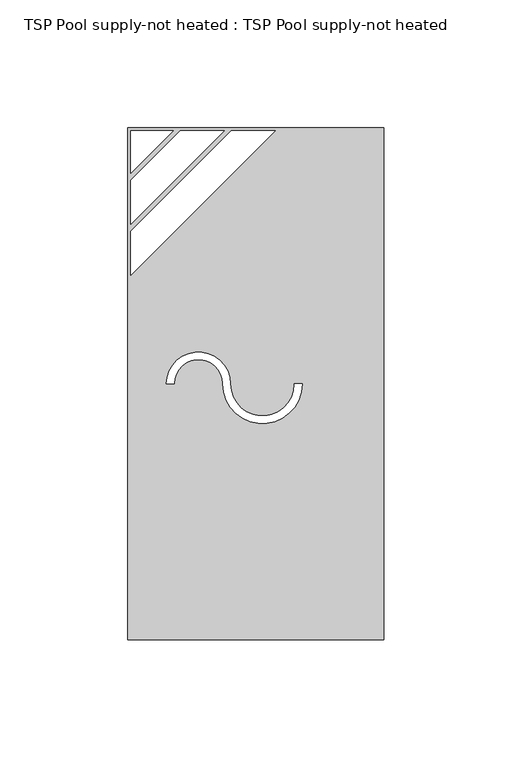
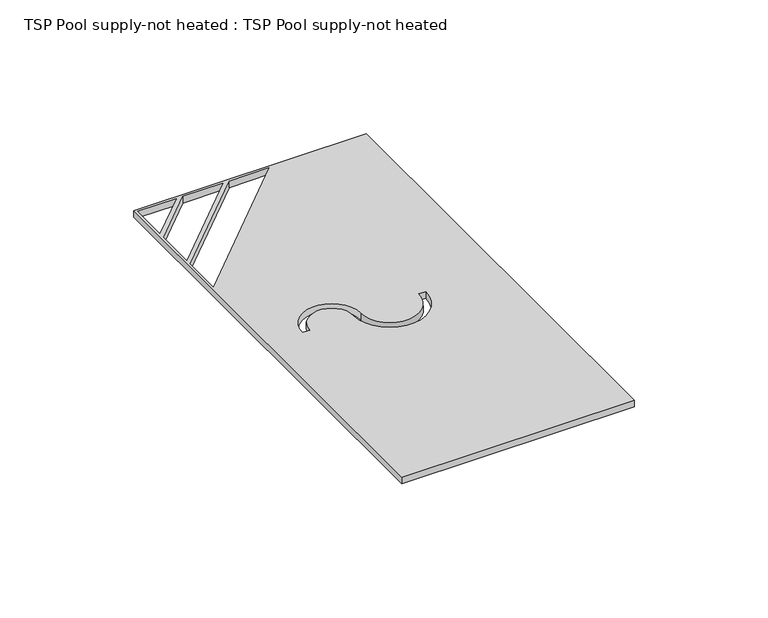
"""IFC4 building model written with IfcOpenShell, lengths in millimetres: proxy geometry, TSP Pool supply-not heated : TSP Pool supply-not heated."""

from ifc_helpers import new_model, si_unit, point, frame_2d, origin, origin_with_axes, place, context, project, spatial, polyline, circle_curve, trimmed, segment, composite_curve, outline, extrude, source, transform, mapped, element, save


def tsp_pool_supply_not_heated_tsp_pool_supply_not_heated_95d609e6(model_context):
    return source(origin(), model_context, "Body", "SweptSolid", [
        extrude(outline(polyline([(-100.0, 100.0), (0.0, 100.0), (0.0, -100.0), (-100.0, -100.0), (-100.0, 100.0)]), holes=[polyline([(-59.5857864, 99.0), (-99.0, 59.5857864), (-99.0, 42.4142136), (-42.4142136, 99.0), (-59.5857864, 99.0)]), polyline([(-99.0, 82.4142136), (-82.4142136, 99.0), (-99.0, 99.0), (-99.0, 82.4142136)]), polyline([(-99.0, 79.5857864), (-99.0, 62.4142136), (-62.4142136, 99.0), (-79.5857864, 99.0), (-99.0, 79.5857864)]), composite_curve([segment(trimmed(circle_curve(frame_2d((-72.5, 0.0)), 9.5), [point((-82.0, 0.0))], [point((-63.0, 0.0))], False, "CARTESIAN"), True, "CONTINUOUS"), segment(trimmed(circle_curve(frame_2d((-47.5, 0.0)), 15.5), [point((-63.0, 0.0))], [point((-32.0, 0.0))], True, "CARTESIAN"), True, "CONTINUOUS"), segment(polyline([(-32.0, 0.0), (-35.0, 0.0)]), True, "CONTINUOUS"), segment(trimmed(circle_curve(frame_2d((-47.5, 0.0)), 12.5), [point((-35.0, 0.0))], [point((-60.0, 0.0))], False, "CARTESIAN"), True, "CONTINUOUS"), segment(trimmed(circle_curve(frame_2d((-72.5, 0.0)), 12.5), [point((-60.0, 0.0))], [point((-85.0, 0.0))], True, "CARTESIAN"), True, "CONTINUOUS"), segment(polyline([(-85.0, 0.0), (-82.0, 0.0)]), True, "CONTINUOUS")], self_intersect=False)]), origin_with_axes(), (0.0, 0.0, 1.0), 3.0),
    ])


if __name__ == "__main__":
    model = new_model("IFC4")
    model_context = context("Model", 3, world=origin())
    ifc_project = project(units=[si_unit("LENGTHUNIT", "METRE", prefix="MILLI")], contexts=[model_context])
    site = spatial("IfcSite", under=ifc_project)
    building = spatial("IfcBuilding", under=site)
    placement = place(None, origin())
    tsp_pool_supply_not_heated_tsp_pool_supply_not_heated_shape = tsp_pool_supply_not_heated_tsp_pool_supply_not_heated_95d609e6(model_context)
    element("IfcBuildingElementProxy", 1, Name="TSP Pool supply-not heated : TSP Pool supply-not heated", ObjectType="TSP Pool supply-not heated : TSP Pool supply-not heated", at=placement, inside=building, context=model_context, shape_type="MappedRepresentation", body=[
        mapped(tsp_pool_supply_not_heated_tsp_pool_supply_not_heated_shape, transform((0.0, 0.0, 0.0), x_axis=(1.0, 0.0, 0.0), y_axis=(0.0, 1.0, 0.0), z_axis=(0.0, 0.0, 1.0))),
    ])
    save(model, "model.ifc")

# Revit data of these elements
# Type "TSP Pool supply-not heated : TSP Pool supply-not heated"
#   Model = "TSP_ELECSPSTD"
#   Default Elevation = 0
# Element 1 (IfcBuildingElementProxy, "TSP Pool supply-not heated : TSP Pool supply-not heated")
#   Materials on its faces: "Plastic, Opaque Black"
# Materials
#   "Plastic, Opaque Black": class "Plastic", colour RGB 0 0 0, transparency 0.7, Description = "Plastic, generic, opaque black", Cost = 0
